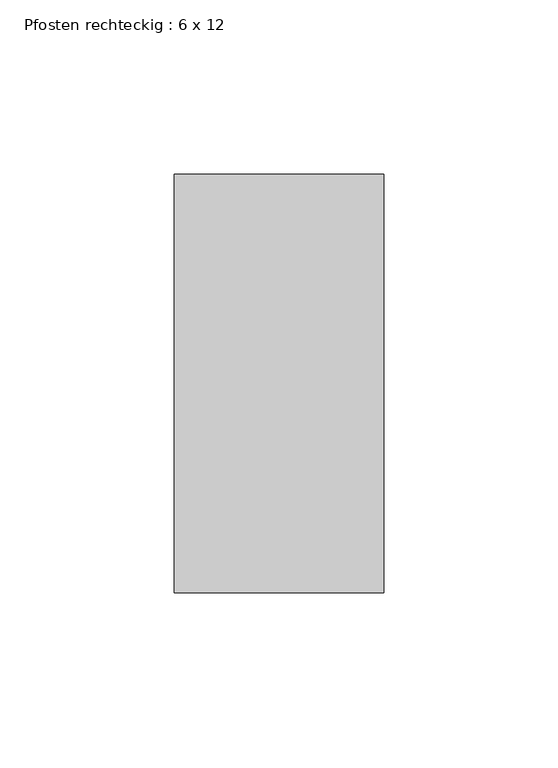
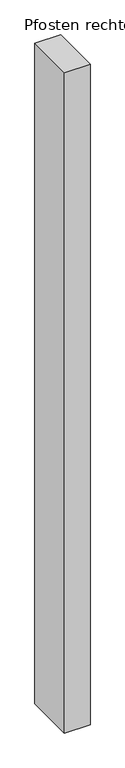
"""IFC4 building model written with IfcOpenShell, lengths in millimetres: member geometry, Pfosten rechteckig : 6 x 12."""

from ifc_helpers import new_model, si_unit, frame, origin, place, context, project, spatial, polyline, outline, extrude, source, transform, mapped, element, save


def pfosten_rechteckig_6_x_12_91242f98(model_context):
    return source(origin(), model_context, "Body", "SweptSolid", [
        extrude(outline(polyline([(0.0, 60.0), (0.0, -60.0), (-60.0, -60.0), (-60.0, 60.0), (0.0, 60.0)])), frame((0.0, 0.0, -1636.6249592), z_axis=(0.0, 0.0, 1.0), x_axis=(1.0, 0.0, 0.0)), (0.0, 0.0, 1.0), 1636.6249592),
    ])


if __name__ == "__main__":
    model = new_model("IFC4")
    model_context = context("Model", 3, world=origin())
    ifc_project = project(units=[si_unit("LENGTHUNIT", "METRE", prefix="MILLI")], contexts=[model_context])
    site = spatial("IfcSite", under=ifc_project)
    building = spatial("IfcBuilding", under=site)
    placement = place(None, origin())
    pfosten_rechteckig_6_x_12_shape = pfosten_rechteckig_6_x_12_91242f98(model_context)
    element("IfcMember", 1, ObjectType="Pfosten rechteckig : 6 x 12", at=placement, inside=building, context=model_context, shape_type="MappedRepresentation", body=[
        mapped(pfosten_rechteckig_6_x_12_shape, transform((0.0, 0.0, 0.0), x_axis=(1.0, 0.0, 0.0), y_axis=(0.0, 1.0, 0.0), z_axis=(0.0, 0.0, 1.0))),
    ])
    save(model, "model.ifc")

# Revit data of these elements
# Type "Pfosten rechteckig : 6 x 12"
#   built-in parameter 1007304 = 0.393701 (stored number, unit not read)
#   built-in parameter 1007301 = 0.0984252 (stored number, unit not read)
#   built-in parameter 1007300 = 0.0984252 (stored number, unit not read)
# Element 1 (IfcMember, "Pfosten rechteckig : 6 x 12")
#   Materials on its faces: "Metall - verzinkt"
# Materials
#   "Metall - verzinkt": class "Allgemeines", colour RGB 200 200 200, transparency 0, Cost = 0
